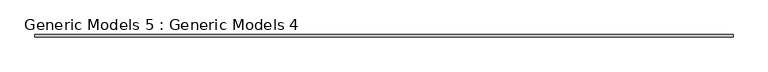
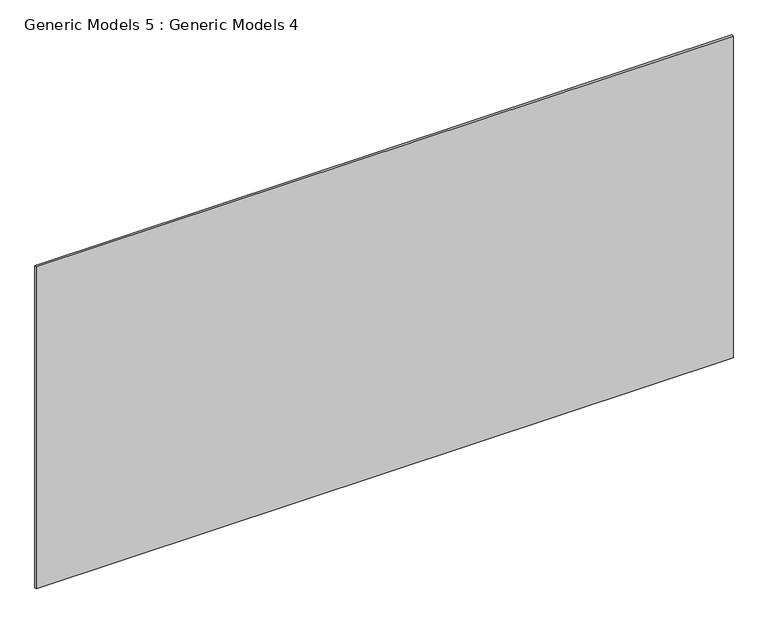
"""IFC4 building model written with IfcOpenShell, lengths in millimetres: proxy geometry, Generic Models 5 : Generic Models 4."""

from ifc_helpers import new_model, si_unit, frame, origin, place, context, project, spatial, polyline, outline, extrude, source, transform, mapped, element, save


def generic_models_5_generic_models_4_a62b5ab6(model_context):
    return source(origin(), model_context, "Body", "SweptSolid", [
        extrude(outline(polyline([(-2310.0733486, -29089.2060818), (-2310.0733486, -29108.2560818), (-8500.0048466, -29108.2560818), (-8500.0048466, -29089.2060818), (-2310.0733486, -29089.2060818)])), frame((0.0, 0.0, 126441.5203834), z_axis=(0.0, 0.0, 1.0), x_axis=(1.0, 0.0, 0.0)), (0.0, 0.0, 1.0), 3021.8229021),
    ])


if __name__ == "__main__":
    model = new_model("IFC4")
    model_context = context("Model", 3, world=origin())
    ifc_project = project(units=[si_unit("LENGTHUNIT", "METRE", prefix="MILLI")], contexts=[model_context])
    site = spatial("IfcSite", under=ifc_project)
    building = spatial("IfcBuilding", under=site)
    placement = place(None, origin())
    generic_models_5_generic_models_4_shape = generic_models_5_generic_models_4_a62b5ab6(model_context)
    element("IfcBuildingElementProxy", 1, Name="Generic Models 5 : Generic Models 4", ObjectType="Generic Models 5 : Generic Models 4", at=placement, inside=building, context=model_context, shape_type="MappedRepresentation", body=[
        mapped(generic_models_5_generic_models_4_shape, transform((0.0, 0.0, 0.0), x_axis=(1.0, 0.0, 0.0), y_axis=(0.0, 1.0, 0.0), z_axis=(0.0, 0.0, 1.0))),
    ])
    save(model, "model.ifc")

# Revit data of these elements
# Element 1 (IfcBuildingElementProxy, "Generic Models 5 : Generic Models 4")
#   Materials on its faces: "_CDX PLYWOOD - SEE STRUCT DWGs"
# Materials
#   "_CDX PLYWOOD - SEE STRUCT DWGs": class "Generic", colour RGB 98 75 74, transparency 0, Cost = 0
